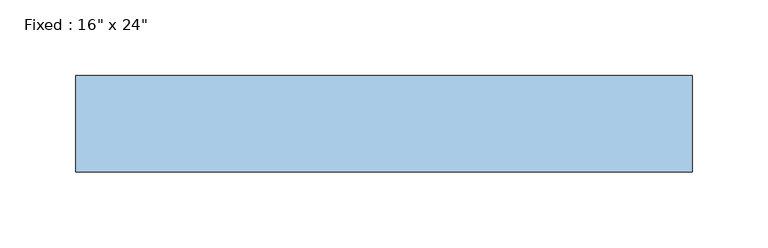
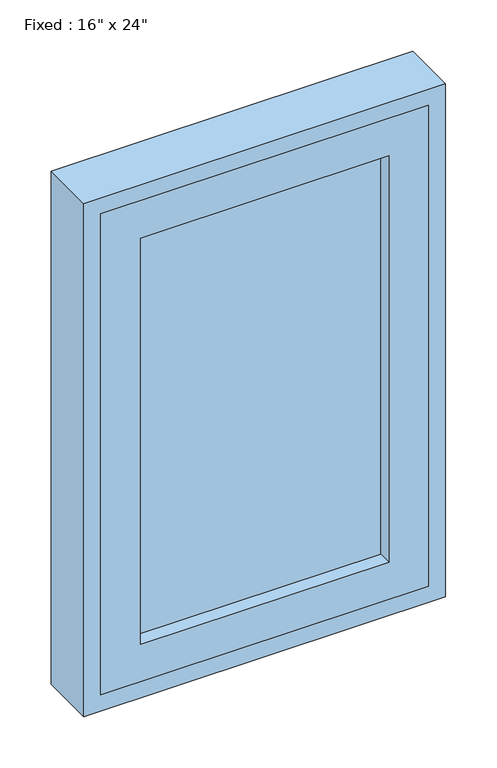
"""IFC4 building model written with IfcOpenShell, lengths in millimetres: window geometry."""

import ifcopenshell
import ifcopenshell.guid

model = None  # the IFC model being written
_history = None  # IfcOwnerHistory: only IFC2X3 demands one
_inside = {}  # id of a spatial element -> (the spatial element, [elements in it])
_under = {}  # id of a project, library or spatial element -> (it, [spatial elements below it])
_declared = {}  # id of a project -> (the project, [libraries it declares])
_typed = {}  # id of a type object -> (the type object, [elements of that type])
_made_of = {}  # id of a material, layer set ... -> (it, [elements and type objects made of it])


def new_model(schema):
    """Start an empty IFC model of exactly this schema.

    Asked for "IFC4X3", IfcOpenShell would pick the latest addendum, in which some entities
    have other attributes; the version numbers below select the first issue.
    IFC2X3 requires an IfcOwnerHistory on every rooted entity: one is made here for all.
    """
    global model, _history
    if schema == "IFC4X3":
        model = ifcopenshell.file(schema_version=(4, 3, 0, 0))
    else:
        model = ifcopenshell.file(schema=schema)
    _inside.clear()
    _under.clear()
    _declared.clear()
    _typed.clear()
    _made_of.clear()
    _history = None
    if model.schema == "IFC2X3":
        org = make("IfcOrganization", Name="unknown")
        user = make(
            "IfcPersonAndOrganization",
            ThePerson=make("IfcPerson", FamilyName="unknown"),
            TheOrganization=org,
        )
        app = make(
            "IfcApplication",
            ApplicationDeveloper=org,
            Version="unknown",
            ApplicationFullName="unknown",
            ApplicationIdentifier="unknown",
        )
        _history = make(
            "IfcOwnerHistory",
            OwningUser=user,
            OwningApplication=app,
            ChangeAction="ADDED",
            CreationDate=0,
        )
    return model


def make(cls, **values):
    """One entity of the class cls with the attributes given. An attribute that is None is left unset."""
    return model.create_entity(
        cls, **{name: value for name, value in values.items() if value is not None}
    )


def rooted(cls, **values):
    """An entity with a GlobalId (a new one), such as an element, a storey or a relation."""
    return make(cls, GlobalId=ifcopenshell.guid.new(), OwnerHistory=_history, **values)


def si_unit(unit_type, name, prefix=None):
    """IfcSIUnit, for example si_unit("LENGTHUNIT", "METRE", prefix="MILLI")."""
    return make("IfcSIUnit", UnitType=unit_type, Prefix=prefix, Name=name)


def assignment(units):
    """IfcUnitAssignment: the units of a project."""
    return None if units is None else make("IfcUnitAssignment", Units=units)


def point(xyz):
    """IfcCartesianPoint."""
    return None if xyz is None else make("IfcCartesianPoint", Coordinates=xyz)


def direction(xyz):
    """IfcDirection."""
    return None if xyz is None else make("IfcDirection", DirectionRatios=xyz)


def frame(location, z_axis=None, x_axis=None):
    """IfcAxis2Placement3D, a coordinate frame: its origin and axes. An axis left out is left unset."""
    return make(
        "IfcAxis2Placement3D",
        Location=point(location),
        Axis=direction(z_axis),
        RefDirection=direction(x_axis),
    )


def origin():
    """The frame at (0, 0, 0) with its axes left unset."""
    return frame((0.0, 0.0, 0.0))


def place(relative_to, where):
    """IfcLocalPlacement: puts the frame where relative to a parent placement (None: the world)."""
    return make(
        "IfcLocalPlacement", PlacementRelTo=relative_to, RelativePlacement=where
    )


def context(
    kind, dimensions, precision=None, world=None, true_north=None, identifier=None
):
    """IfcGeometricRepresentationContext, for example the 3D "Model" context."""
    return make(
        "IfcGeometricRepresentationContext",
        ContextIdentifier=identifier,
        ContextType=kind,
        CoordinateSpaceDimension=dimensions,
        Precision=precision,
        WorldCoordinateSystem=world,
        TrueNorth=true_north,
    )


def project(units=None, contexts=None):
    """IfcProject with its units and contexts."""
    return rooted(
        "IfcProject",
        Name="project",
        RepresentationContexts=contexts,
        UnitsInContext=assignment(units),
    )


def spatial(cls, under=None, at=None, **own):
    """A site, building, storey or space (cls), placed at a placement, below another one or the project."""
    s = rooted(cls, ObjectPlacement=at, **own)
    if under is not None:
        _under.setdefault(under.id(), (under, []))[1].append(s)
    return s


def polyline(points):
    """IfcPolyline through the points."""
    return make("IfcPolyline", Points=[point(p) for p in points])


def outline(outer, holes=None, kind="AREA"):
    """IfcArbitraryClosedProfileDef: a profile drawn as a closed curve; with holes, ...WithVoids."""
    if holes is None:
        return make("IfcArbitraryClosedProfileDef", ProfileType=kind, OuterCurve=outer)
    return make(
        "IfcArbitraryProfileDefWithVoids",
        ProfileType=kind,
        OuterCurve=outer,
        InnerCurves=holes,
    )


def extrude(swept, where, along, depth):
    """IfcExtrudedAreaSolid: the profile swept, set in the frame where, extruded along a direction by depth."""
    return make(
        "IfcExtrudedAreaSolid",
        SweptArea=swept,
        Position=where,
        ExtrudedDirection=direction(along),
        Depth=depth,
    )


def shape(context_of_items, identifier, shape_type, items):
    """IfcShapeRepresentation: the items that make up one representation, for example the "Body"."""
    return make(
        "IfcShapeRepresentation",
        ContextOfItems=context_of_items,
        RepresentationIdentifier=identifier,
        RepresentationType=shape_type,
        Items=items,
    )


def source(mapping_origin, context_of_items, identifier, shape_type, items):
    """IfcRepresentationMap: a shape defined once, which mapped items show again and again."""
    return make(
        "IfcRepresentationMap",
        MappingOrigin=mapping_origin,
        MappedRepresentation=shape(context_of_items, identifier, shape_type, items),
    )


def transform(
    local_origin,
    x_axis=None,
    y_axis=None,
    z_axis=None,
    scale=None,
    scale2=None,
    scale3=None,
    uniform=True,
):
    """IfcCartesianTransformationOperator3D, or its non-uniform kind. x_axis, y_axis, z_axis: its Axis1, 2, 3."""
    if uniform:
        return make(
            "IfcCartesianTransformationOperator3D",
            Axis1=direction(x_axis),
            Axis2=direction(y_axis),
            LocalOrigin=point(local_origin),
            Scale=scale,
            Axis3=direction(z_axis),
        )
    return make(
        "IfcCartesianTransformationOperator3DnonUniform",
        Axis1=direction(x_axis),
        Axis2=direction(y_axis),
        LocalOrigin=point(local_origin),
        Scale=scale,
        Axis3=direction(z_axis),
        Scale2=scale2,
        Scale3=scale3,
    )


def mapped(mapping_source, mapping_target):
    """IfcMappedItem: shows the shape of a source again, moved by a transform."""
    return make(
        "IfcMappedItem", MappingSource=mapping_source, MappingTarget=mapping_target
    )


def made_of(thing, what):
    """Note that an element or type object is made of a material, layer set ...; save() writes the relation."""
    if what is not None:
        _made_of.setdefault(what.id(), (what, []))[1].append(thing)
    return thing


def element(
    cls,
    number,
    at=None,
    inside=None,
    cuts=None,
    type_object=None,
    material=None,
    context=None,
    identifier="Body",
    shape_type=None,
    held_by="IfcProductDefinitionShape",
    body=None,
    shapes=None,
    **own,
):
    """One element of the class cls, such as IfcWall. Its Tag is "e" and its number.

    at: its placement. inside: the storey or other place that contains it. cuts: it is an
    opening in that element (IfcRelVoidsElement). A single representation is given by context,
    identifier, shape_type and body (its items); several are given by shapes. held_by: the class
    of the entity that holds the representations. save() writes the other relations.
    """
    e = rooted(cls, Tag="e%d" % number, ObjectPlacement=at, **own)
    if body is not None:
        shapes = [shape(context, identifier, shape_type, body)]
    if shapes is not None:
        e.Representation = make(held_by, Representations=shapes)
    if inside is not None:
        _inside.setdefault(inside.id(), (inside, []))[1].append(e)
    if cuts is not None:
        rooted(
            "IfcRelVoidsElement", RelatingBuildingElement=cuts, RelatedOpeningElement=e
        )
    if type_object is not None:
        _typed.setdefault(type_object.id(), (type_object, []))[1].append(e)
    return made_of(e, material)


def aggregate(whole, parts):
    """IfcRelAggregates: a whole, such as a stair, and the parts it consists of."""
    return rooted("IfcRelAggregates", RelatingObject=whole, RelatedObjects=parts)


def save(model, path):
    """Write the relations noted so far, then the file.

    IfcRelAggregates (storeys below a building ...), IfcRelContainedInSpatialStructure (elements
    in a storey), IfcRelDefinesByType, IfcRelAssociatesMaterial and IfcRelDeclares: one each for
    every whole, place, type object, material and project.
    """
    for whole, parts in _under.values():
        aggregate(whole, parts)
    for where, things in _inside.values():
        rooted(
            "IfcRelContainedInSpatialStructure",
            RelatedElements=things,
            RelatingStructure=where,
        )
    for kind, things in _typed.values():
        rooted("IfcRelDefinesByType", RelatedObjects=things, RelatingType=kind)
    for what, things in _made_of.values():
        rooted("IfcRelAssociatesMaterial", RelatedObjects=things, RelatingMaterial=what)
    for by, libraries in _declared.values():
        rooted("IfcRelDeclares", RelatingContext=by, RelatedDefinitions=libraries)
    model.write(path)


def window_b0fd0360(model_context):
    return source(origin(), model_context, "Body", "SweptSolid", [
        extrude(outline(polyline([(101.6, -15.875), (-177.8, -15.875), (-177.8, -3.175), (101.6, -3.175), (101.6, -15.875)])), frame((0.0, 0.0, 977.9), z_axis=(0.0, 0.0, 1.0), x_axis=(1.0, 0.0, 0.0)), (0.0, 0.0, 1.0), 482.6),
        extrude(outline(polyline([(1504.95, -222.25), (933.45, -222.25), (933.45, 146.05), (1504.95, 146.05), (1504.95, -222.25)]), holes=[polyline([(1460.5, -177.8), (1460.5, 101.6), (977.9, 101.6), (977.9, -177.8), (1460.5, -177.8)])]), frame((0.0, -31.75, 0.0), z_axis=(0.0, 1.0, 0.0), x_axis=(0.0, 0.0, 1.0)), (0.0, 0.0, 1.0), 44.45),
        extrude(outline(polyline([(1524.0, 165.1), (1524.0, -241.3), (914.4, -241.3), (914.4, 165.1), (1524.0, 165.1)]), holes=[polyline([(1504.95, 146.05), (933.45, 146.05), (933.45, -222.25), (1504.95, -222.25), (1504.95, 146.05)])]), frame((0.0, -31.75, 0.0), z_axis=(0.0, 1.0, 0.0), x_axis=(0.0, 0.0, 1.0)), (0.0, 0.0, 1.0), 63.5),
    ])


if __name__ == "__main__":
    model = new_model("IFC4")
    model_context = context("Model", 3, world=origin())
    ifc_project = project(units=[si_unit("LENGTHUNIT", "METRE", prefix="MILLI")], contexts=[model_context])
    site = spatial("IfcSite", under=ifc_project)
    building = spatial("IfcBuilding", under=site)
    placement = place(None, origin())
    window_shape = window_b0fd0360(model_context)
    element("IfcWindow", 1, ObjectType="Fixed : 16\" x 24\"", at=placement, inside=building, context=model_context, shape_type="MappedRepresentation", body=[
        mapped(window_shape, transform((0.0, 0.0, 0.0), x_axis=(1.0, 0.0, 0.0), y_axis=(0.0, 1.0, 0.0), z_axis=(0.0, 0.0, 1.0))),
    ])
    save(model, "model.ifc")

# Revit data of these elements
# Type "Fixed : 16\" x 24\""
#   Type Mark = "4"
#   Construction Type Id = "GSP4R"
#   Assembly Code = "B2020100"
#   Analytic Construction = "1/8 in Pilkington single glazing"
#   Visual Light Transmittance = 0.9
#   Solar Heat Gain Coefficient = 0.78
#   Heat Transfer Coefficient (U) = 0.6496 BTU/(h·ft²·°F)
#   Height = 2' - 0"
#   Default Sill Height = 3' - 0"
#   Width = 1' - 4"
#   Window Inset = 0' - 0 3/4"
#   Define Thermal Properties by = 1
#   Define Thermal Properties by = 1
#   Glass Pane Material = Glass
#   Sash Material = Sash
#   Wall Closure = (empty or 0)
# Element 1 (IfcWindow, "Fixed : 16\" x 24\"")
#   Materials on its faces: "Sash", "Glass"
# Materials
#   "Glass": class "Glass", colour RGB 0 128 192, transparency 0.75, Description = "Soda Lime Glass", Cost = 0
#   "Sash": class "Wood", colour RGB 224 178 126, transparency 0, Cost = 0
